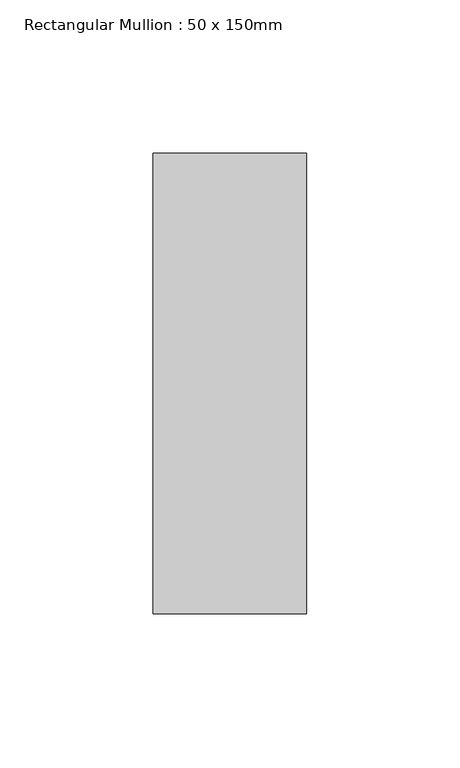
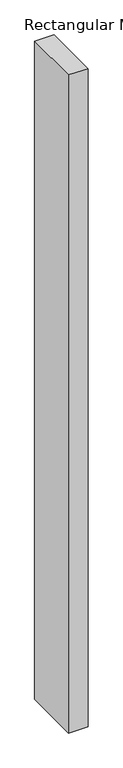
"""IFC4 building model written with IfcOpenShell, lengths in millimetres: member geometry, Rectangular Mullion : 50 x 150mm."""

from ifc_helpers import new_model, si_unit, frame, origin, place, context, project, spatial, polyline, outline, extrude, source, transform, mapped, element, save


def rectangular_mullion_50_x_150mm_ca8dd098(model_context):
    return source(origin(), model_context, "Body", "SweptSolid", [
        extrude(outline(polyline([(25.0, 75.0), (25.0, -75.0), (-25.0, -75.0), (-25.0, 75.0), (25.0, 75.0)])), frame((0.0, 0.0, -1782.0), z_axis=(0.0, 0.0, 1.0), x_axis=(1.0, 0.0, 0.0)), (0.0, 0.0, 1.0), 1782.0),
    ])


if __name__ == "__main__":
    model = new_model("IFC4")
    model_context = context("Model", 3, world=origin())
    ifc_project = project(units=[si_unit("LENGTHUNIT", "METRE", prefix="MILLI")], contexts=[model_context])
    site = spatial("IfcSite", under=ifc_project)
    building = spatial("IfcBuilding", under=site)
    placement = place(None, origin())
    rectangular_mullion_50_x_150mm_shape = rectangular_mullion_50_x_150mm_ca8dd098(model_context)
    element("IfcMember", 1, ObjectType="Rectangular Mullion : 50 x 150mm", at=placement, inside=building, context=model_context, shape_type="MappedRepresentation", body=[
        mapped(rectangular_mullion_50_x_150mm_shape, transform((0.0, 0.0, 0.0), x_axis=(1.0, 0.0, 0.0), y_axis=(0.0, 1.0, 0.0), z_axis=(0.0, 0.0, 1.0))),
    ])
    save(model, "model.ifc")

# Revit data of these elements
# Type "Rectangular Mullion : 50 x 150mm"
#   Keynote = "H11"
#   built-in parameter 1007304 = 0.492126 (stored number, unit not read)
#   built-in parameter 1007301 = 0.082021 (stored number, unit not read)
#   built-in parameter 1007300 = 0.082021 (stored number, unit not read)
# Element 1 (IfcMember, "Rectangular Mullion : 50 x 150mm")
#   Materials on its faces: "Aluminium"
# Materials
#   "Aluminium": class "Metal", colour RGB 247 247 247, transparency 0, Description = "Aluminium 6061", Cost = 0
